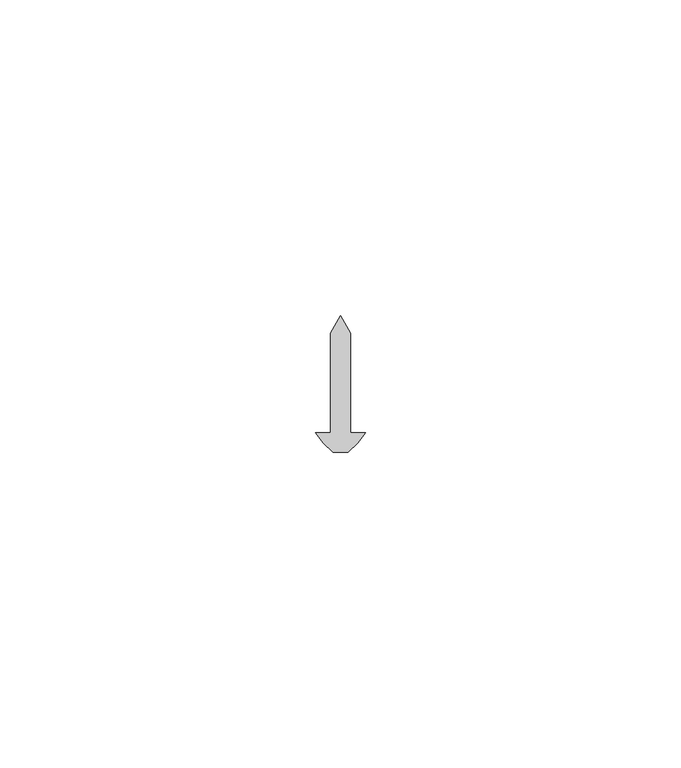
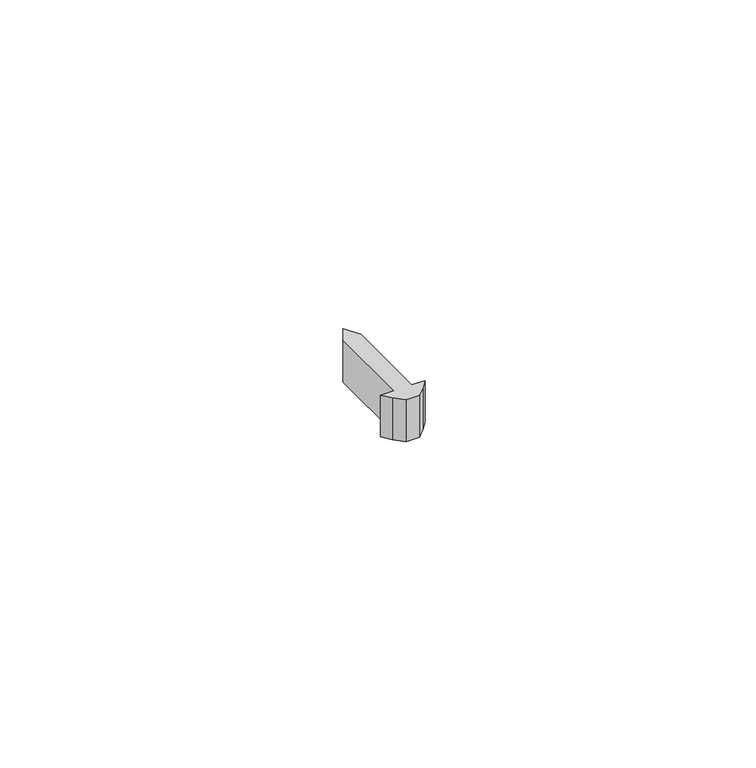
"""IFC4 building model written with IfcOpenShell, lengths in millimetres: proxy geometry, Generic Models 7:Generic Models 1:3:Generic Models 1:3 : Generic Models 7:Generic Models 1:305549:3:Generic Models 1:3:Generic Models 1:3 : Generic Models 7:Generic Models 1:305549:3 : Generic Models 7:Generic Models 1:3:Generic Models 1:3 : Generic Models 7:Generic Models 1:305549:301244:3 : Generic Models 7:Generic Models 1:3:Generic Models 1:3 : Generic Models 7:Generic Models 1:305549:3:Generic Models 1:3:Generic Models 1:3 : Generic Models 7:Generic Models 1:305549:3 : Generic Models 7:Generic Models 1:3:Generic Models 1:3 : Generic Models 7:Generic Models 1:305549:301244:308848."""

from ifc_helpers import new_model, si_unit, frame, origin, place, context, project, spatial, polyline, outline, extrude, source, transform, mapped, element, save


def generic_models_80caf22e(model_context):
    return source(origin(), model_context, "Body", "SweptSolid", [
        extrude(outline(polyline([(594923.9492239, -579084.8288841), (594923.9492239, -579069.0196286), (594925.5367239, -579066.2699979), (594927.1242239, -579069.0196286), (594927.1242239, -579084.8288841), (594929.5054739, -579084.8288841), (594928.2872784, -579086.3559421), (594926.7353882, -579087.9078323), (594924.3380597, -579087.9078323), (594922.7861695, -579086.3559421), (594921.5679739, -579084.8288841), (594923.9492239, -579084.8288841)])), frame((0.0, 0.0, 1237.45625), z_axis=(0.0, 0.0, 1.0), x_axis=(1.0, 0.0, 0.0)), (0.0, 0.0, 1.0), 7.9375),
    ])


if __name__ == "__main__":
    model = new_model("IFC4")
    model_context = context("Model", 3, world=origin())
    ifc_project = project(units=[si_unit("LENGTHUNIT", "METRE", prefix="MILLI")], contexts=[model_context])
    site = spatial("IfcSite", under=ifc_project)
    building = spatial("IfcBuilding", under=site)
    placement = place(None, origin())
    generic_models_shape = generic_models_80caf22e(model_context)
    element("IfcBuildingElementProxy", 1, Name="Generic Models 7:Generic Models 1:3:Generic Models 1:3 : Generic Models 7:Generic Models 1:305549:3:Generic Models 1:3:Generic Models 1:3 : Generic Models 7:Generic Models 1:305549:3 : Generic Models 7:Generic Models 1:3:Generic Models 1:3 : Generic Models 7:Generic Models 1:305549:301244:3 : Generic Models 7:Generic Models 1:3:Generic Models 1:3 : Generic Models 7:Generic Models 1:305549:3:Generic Models 1:3:Generic Models 1:3 : Generic Models 7:Generic Models 1:305549:3 : Generic Models 7:Generic Models 1:3:Generic Models 1:3 : Generic Models 7:Generic Models 1:305549:301244:308848", ObjectType="Generic Models 7:Generic Models 1:3:Generic Models 1:3 : Generic Models 7:Generic Models 1:305549:3:Generic Models 1:3:Generic Models 1:3 : Generic Models 7:Generic Models 1:305549:3 : Generic Models 7:Generic Models 1:3:Generic Models 1:3 : Generic Models 7:Generic Models 1:305549:301244:3 : Generic Models 7:Generic Models 1:3:Generic Models 1:3 : Generic Models 7:Generic Models 1:305549:3:Generic Models 1:3:Generic Models 1:3 : Generic Models 7:Generic Models 1:305549:3 : Generic Models 7:Generic Models 1:3:Generic Models 1:3 : Generic Models 7:Generic Models 1:305549:301244:308848", at=placement, inside=building, context=model_context, shape_type="MappedRepresentation", body=[
        mapped(generic_models_shape, transform((0.0, 0.0, 0.0), x_axis=(1.0, 0.0, 0.0), y_axis=(0.0, 1.0, 0.0), z_axis=(0.0, 0.0, 1.0))),
    ])
    save(model, "model.ifc")

# Revit data of these elements
# Type "Generic Models 7:Generic Models 1:3:Generic Models 1:3 : Generic Models 7:Generic Models 1:305549:3:Generic Models 1:3:Generic Models 1:3 : Generic Models 7:Generic Models 1:305549:3 : Generic Models 7:Generic Models 1:3:Generic Models 1:3 : Generic Models 7:Generic Models 1:305549:301244:3 : Generic Models 7:Generic Models 1:3:Generic Models 1:3 : Generic Models 7:Generic Models 1:305549:3:Generic Models 1:3:Generic Models 1:3 : Generic Models 7:Generic Models 1:305549:3 : Generic Models 7:Generic Models 1:3:Generic Models 1:3 : Generic Models 7:Generic Models 1:305549:301244:308848"
#   NameOverride = "Generic Models 7:Generic Models 1:3:Generic Models 1:3 : Generic Models 7:Generic Models 1:305549:3:Generic Models 1:3:Generic Models 1:3 : Generic Models 7:Generic Models 1:305549:3 : Generic Models 7:Generic Models 1:3:Generic Models 1:3 : Generic Models 7:Generic Models 1:305549:301244:308848"
#   ObjectTypeOverride = "Generic Models 1:3:Generic Models 1:3 : Generic Models 7:Generic Models 1:305549:3 : Generic Models 7:Generic Models 1:3:Generic Models 1:3 : Generic Models 7:Generic Models 1:305549:301244"
#   Reference = "Generic Models 1"
#   Tag = "308848"
# Element 1 (IfcBuildingElementProxy, "Generic Models 7:Generic Models 1:3:Generic Models 1:3 : Generic Models 7:Generic Models 1:305549:3:Generic Models 1:3:Generic Models 1:3 : Generic Models 7:Generic Models 1:305549:3 : Generic Models 7:Generic Models 1:3:Generic Models 1:3 : Generic Models 7:Generic Models 1:305549:301244:3 : Generic Models 7:Generic Models 1:3:Generic Models 1:3 : Generic Models 7:Generic Models 1:305549:3:Generic Models 1:3:Generic Models 1:3 : Generic Models 7:Generic Models 1:305549:3 : Generic Models 7:Generic Models 1:3:Generic Models 1:3 : Generic Models 7:Generic Models 1:305549:301244:308848")
#   Materials on its faces: "FASTENERS (T.B.D)"
# Materials
#   "FASTENERS (T.B.D)": class "Generic", colour RGB 120 120 120, transparency 0, Cost = 0
